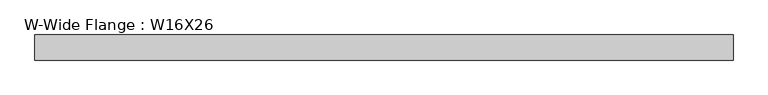
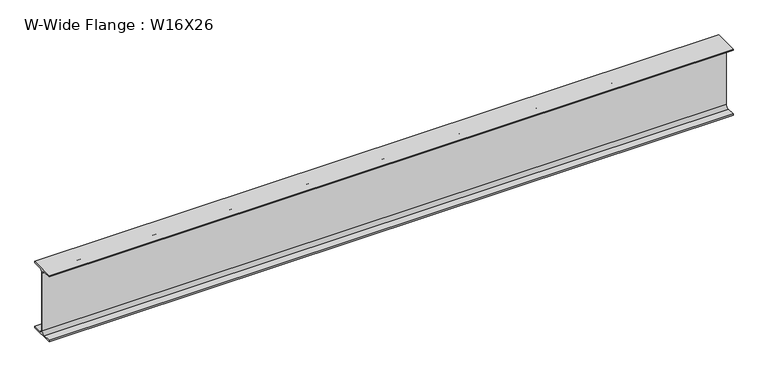
"""IFC4 building model written with IfcOpenShell, lengths in millimetres: beam geometry, W-Wide Flange : W16X26."""

from ifc_helpers import new_model, si_unit, point, frame, frame_2d, origin, place, context, project, spatial, polyline, circle_curve, trimmed, segment, composite_curve, outline, extrude, source, transform, mapped, element, save


def w_wide_flange_w16x26_e9865469(model_context):
    return source(origin(), model_context, "Body", "SweptSolid", [
        extrude(outline(composite_curve([segment(polyline([(69.85, -190.627), (69.85, -199.39), (-69.85, -199.39), (-69.85, -190.627), (-21.3995, -190.627)]), True, "CONTINUOUS"), segment(trimmed(circle_curve(frame_2d((-21.3995, -172.4025)), 18.2245), [point((-21.3995, -190.627))], [point((-3.175, -172.4025))], True, "CARTESIAN"), True, "CONTINUOUS"), segment(polyline([(-3.175, -172.4025), (-3.175, 172.4025)]), True, "CONTINUOUS"), segment(trimmed(circle_curve(frame_2d((-21.3995, 172.4025)), 18.2245), [point((-3.175, 172.4025))], [point((-21.3995, 190.627))], True, "CARTESIAN"), True, "CONTINUOUS"), segment(polyline([(-21.3995, 190.627), (-69.85, 190.627), (-69.85, 199.39), (69.85, 199.39), (69.85, 190.627), (21.3995, 190.627)]), True, "CONTINUOUS"), segment(trimmed(circle_curve(frame_2d((21.3995, 172.4025)), 18.2245), [point((21.3995, 190.627))], [point((3.175, 172.4025))], True, "CARTESIAN"), True, "CONTINUOUS"), segment(polyline([(3.175, 172.4025), (3.175, -172.4025)]), True, "CONTINUOUS"), segment(trimmed(circle_curve(frame_2d((21.3995, -172.4025)), 18.2245), [point((3.175, -172.4025))], [point((21.3995, -190.627))], True, "CARTESIAN"), True, "CONTINUOUS"), segment(polyline([(21.3995, -190.627), (69.85, -190.627)]), True, "CONTINUOUS")], self_intersect=False)), frame((-1981.2, 0.0, 0.0), z_axis=(1.0, 0.0, 0.0), x_axis=(0.0, 1.0, 0.0)), (0.0, 0.0, 1.0), 3886.2),
    ])


if __name__ == "__main__":
    model = new_model("IFC4")
    model_context = context("Model", 3, world=origin())
    ifc_project = project(units=[si_unit("LENGTHUNIT", "METRE", prefix="MILLI")], contexts=[model_context])
    site = spatial("IfcSite", under=ifc_project)
    building = spatial("IfcBuilding", under=site)
    placement = place(None, origin())
    w_wide_flange_w16x26_shape = w_wide_flange_w16x26_e9865469(model_context)
    element("IfcBeam", 1, ObjectType="W-Wide Flange : W16X26", at=placement, inside=building, context=model_context, shape_type="MappedRepresentation", body=[
        mapped(w_wide_flange_w16x26_shape, transform((0.0, 0.0, 0.0), x_axis=(1.0, 0.0, 0.0), y_axis=(0.0, 1.0, 0.0), z_axis=(0.0, 0.0, 1.0))),
    ])
    save(model, "model.ifc")

# Revit data of these elements
# Type "W-Wide Flange : W16X26"
#   Assembly Code = "B10"
#   W = 26
#   Length [instance default] = 5' - 0"
#   bf = 0' - 5 1/2"
#   d = 1' - 3.7"
#   k = 0' - 1 1/16"
#   k2 = 0' - 0.7175"
#   tf = 0' - 0.345"
#   tw = 0' - 0 1/4"
#   A = 0.0533333 SF
#   Structural Material [instance default] = Steel ASTM A992
# Element 1 (IfcBeam, "W-Wide Flange : W16X26")
#   Structural Material = Steel ASTM A36
#   Materials on its faces: "Steel ASTM A36"
# Materials
#   "Steel ASTM A992": class "Metal", colour RGB 199 199 199, transparency 0, Description = "Structural steel 50ksi", Cost = 0
#   "Steel ASTM A36": class "Metal", colour RGB 199 199 199, transparency 0, Description = "Structural steel, ASTM A36 Grade B, mill finish", Cost = 0
